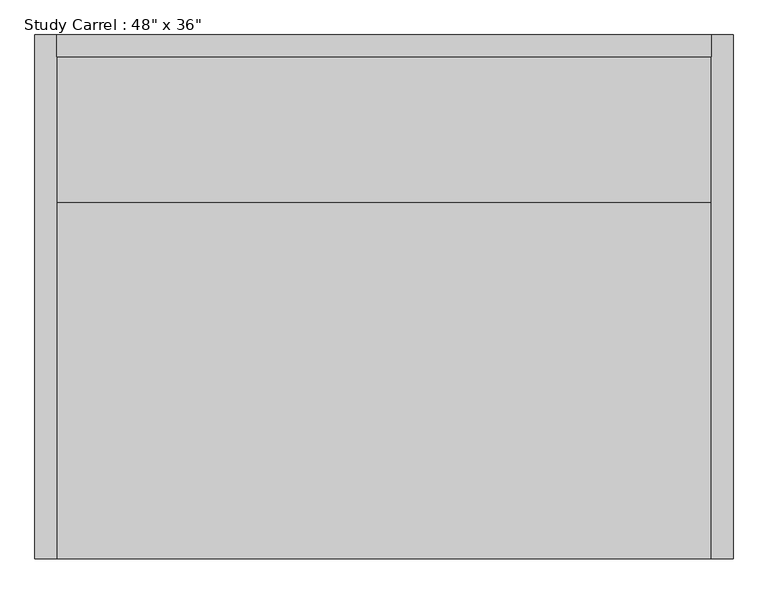
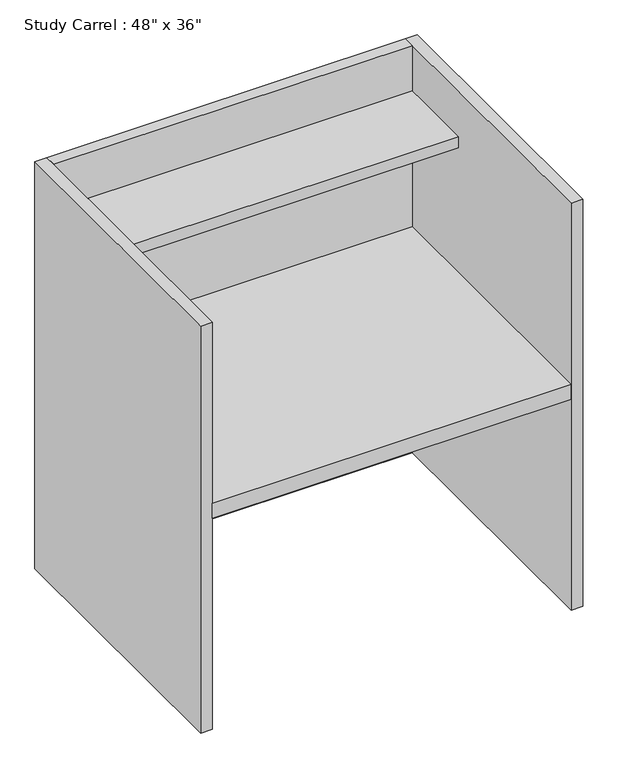
"""IFC4 building model written with IfcOpenShell, lengths in millimetres: furniture geometry."""

from ifc_helpers import new_model, si_unit, frame, origin, origin_with_axes, place, context, project, spatial, polyline, outline, extrude, source, transform, mapped, element, save


def furniture_f3bb4c7c(model_context):
    return source(origin(), model_context, "Body", "SweptSolid", [
        extrude(outline(polyline([(571.5, 419.1), (571.5, -457.2), (-571.5, -457.2), (-571.5, 419.1), (571.5, 419.1)])), frame((0.0, 0.0, 711.2), z_axis=(0.0, 0.0, 1.0), x_axis=(1.0, 0.0, 0.0)), (0.0, 0.0, 1.0), 50.8),
        extrude(outline(polyline([(571.5, 419.1), (571.5, 165.1), (-571.5, 165.1), (-571.5, 419.1), (571.5, 419.1)])), frame((0.0, 0.0, 1181.1), z_axis=(0.0, 0.0, 1.0), x_axis=(1.0, 0.0, 0.0)), (0.0, 0.0, 1.0), 38.1),
        extrude(outline(polyline([(571.5, 419.1), (-571.5, 419.1), (-571.5, 457.2), (571.5, 457.2), (571.5, 419.1)])), origin_with_axes(), (0.0, 0.0, 1.0), 1371.6),
        extrude(outline(polyline([(609.6, 457.2), (609.6, -457.2), (571.5, -457.2), (571.5, 457.2), (609.6, 457.2)])), origin_with_axes(), (0.0, 0.0, 1.0), 1371.6),
        extrude(outline(polyline([(-571.5, -457.2), (-609.6, -457.2), (-609.6, 457.2), (-571.5, 457.2), (-571.5, -457.2)])), origin_with_axes(), (0.0, 0.0, 1.0), 1371.6),
    ])


if __name__ == "__main__":
    model = new_model("IFC4")
    model_context = context("Model", 3, world=origin())
    ifc_project = project(units=[si_unit("LENGTHUNIT", "METRE", prefix="MILLI")], contexts=[model_context])
    site = spatial("IfcSite", under=ifc_project)
    building = spatial("IfcBuilding", under=site)
    placement = place(None, origin())
    furniture_shape = furniture_f3bb4c7c(model_context)
    element("IfcFurniture", 1, ObjectType="Study Carrel : 48\" x 36\"", at=placement, inside=building, context=model_context, shape_type="MappedRepresentation", body=[
        mapped(furniture_shape, transform((0.0, 0.0, 0.0), x_axis=(1.0, 0.0, 0.0), y_axis=(0.0, 1.0, 0.0), z_axis=(0.0, 0.0, 1.0))),
    ])
    save(model, "model.ifc")

# Revit data of these elements
# Type "Study Carrel : 48\" x 36\""
#   Assembly Code = "E2020"
#   Depth = 3' - 0"
#   Height = 4' - 6"
#   Width = 4' - 0"
#   Finish = Wood - Birch
#   Default Elevation = 0
# Element 1 (IfcFurniture, "Study Carrel : 48\" x 36\"")
#   Materials on its faces: "Wood - Birch"
# Materials
#   "Wood - Birch": class "Unassigned", colour RGB 224 178 126, transparency 0
